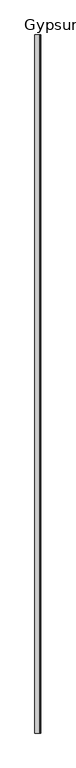
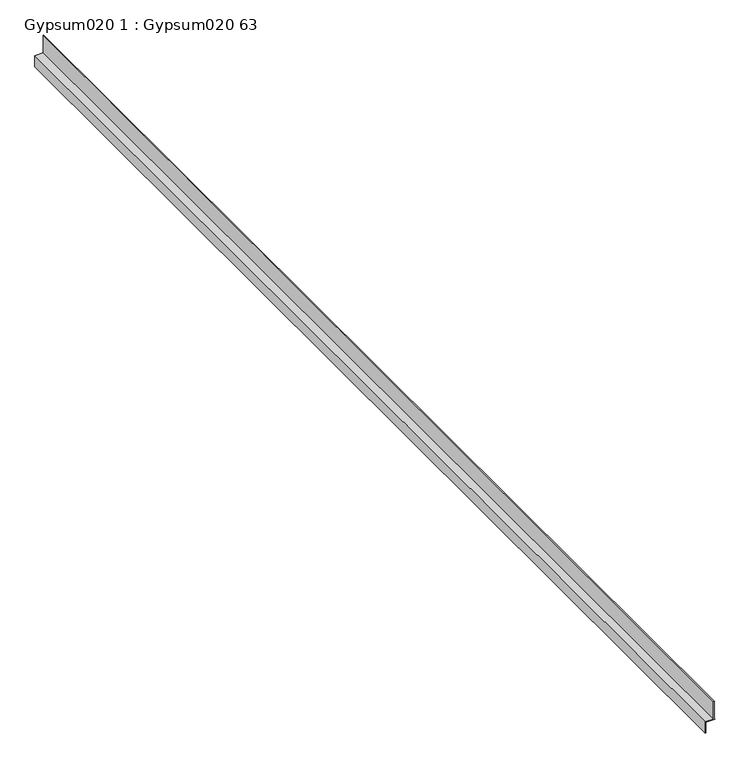
"""IFC4 building model written with IfcOpenShell, lengths in millimetres: proxy geometry, Gypsum020 1 : Gypsum020 63."""

from ifc_helpers import new_model, si_unit, frame, origin, place, context, project, spatial, polyline, outline, extrude, source, transform, mapped, element, save


def gypsum020_1_gypsum020_63_4eaf3a01(model_context):
    return source(origin(), model_context, "Body", "SweptSolid", [
        extrude(outline(polyline([(32619.6960253, -9500.3037014), (32638.7960253, -9500.3037014), (32638.7960253, -9485.2056148), (32640.0660253, -9485.2056148), (32640.0660253, -9486.0154619), (32671.8160253, -9486.0154619), (32671.8160253, -9487.2854619), (32640.0660253, -9487.2854619), (32640.0660253, -9501.5737014), (32619.6960253, -9501.5737014), (32619.6960253, -9500.3037014)])), frame((0.0, 7182.1529373, 0.0), z_axis=(0.0, 1.0, 0.0), x_axis=(0.0, 0.0, 1.0)), (0.0, 0.0, 1.0), 2000.0),
    ])


if __name__ == "__main__":
    model = new_model("IFC4")
    model_context = context("Model", 3, world=origin())
    ifc_project = project(units=[si_unit("LENGTHUNIT", "METRE", prefix="MILLI")], contexts=[model_context])
    site = spatial("IfcSite", under=ifc_project)
    building = spatial("IfcBuilding", under=site)
    placement = place(None, origin())
    gypsum020_1_gypsum020_63_shape = gypsum020_1_gypsum020_63_4eaf3a01(model_context)
    element("IfcBuildingElementProxy", 1, Name="Gypsum020 1 : Gypsum020 63", ObjectType="Gypsum020 1 : Gypsum020 63", at=placement, inside=building, context=model_context, shape_type="MappedRepresentation", body=[
        mapped(gypsum020_1_gypsum020_63_shape, transform((0.0, 0.0, 0.0), x_axis=(1.0, 0.0, 0.0), y_axis=(0.0, 1.0, 0.0), z_axis=(0.0, 0.0, 1.0))),
    ])
    save(model, "model.ifc")

# Revit data of these elements
# Type "Gypsum020 1 : Gypsum020 63"
#   NameOverride = "Gypsum020"
# Element 1 (IfcBuildingElementProxy, "Gypsum020 1 : Gypsum020 63")
#   Materials on its faces: "SHADOW Z REVEAL  BEAD"
# Materials
#   "SHADOW Z REVEAL  BEAD": class "Unassigned", colour RGB 251 232 155, transparency 0, Cost = 0
